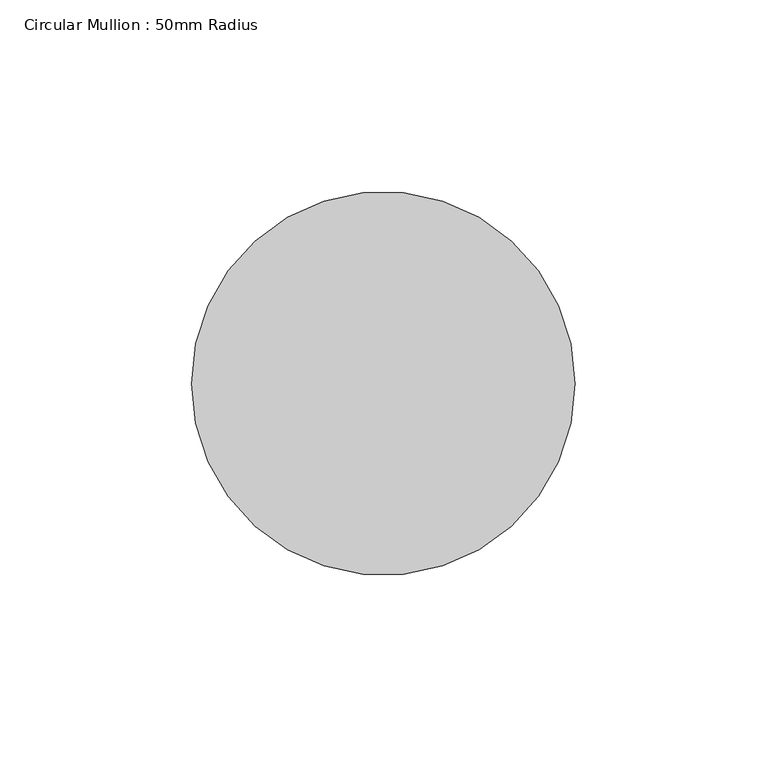
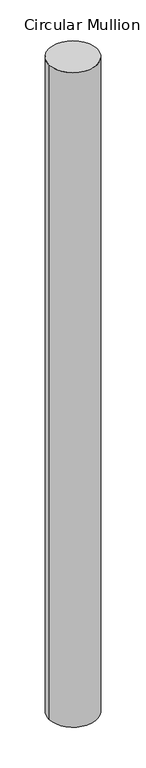
"""IFC4 building model written with IfcOpenShell, lengths in millimetres: member geometry, Circular Mullion : 50mm Radius."""

from ifc_helpers import new_model, si_unit, point, frame, origin, origin_2d, place, context, project, spatial, circle_curve, trimmed, segment, composite_curve, outline, extrude, source, transform, mapped, element, save


def circular_mullion_50mm_radius_7d129db9(model_context):
    return source(origin(), model_context, "Body", "SweptSolid", [
        extrude(outline(composite_curve([segment(trimmed(circle_curve(origin_2d(), 50.0), [point((50.0, 0.0))], [point((-50.0, 0.0))], False, "CARTESIAN"), True, "CONTINUOUS"), segment(trimmed(circle_curve(origin_2d(), 50.0), [point((-50.0, 0.0))], [point((50.0, 0.0))], False, "CARTESIAN"), True, "CONTINUOUS")], self_intersect=False)), frame((0.0, 0.0, -1433.6464214), z_axis=(0.0, 0.0, 1.0), x_axis=(1.0, 0.0, 0.0)), (0.0, 0.0, 1.0), 1433.6464214),
    ])


if __name__ == "__main__":
    model = new_model("IFC4")
    model_context = context("Model", 3, world=origin())
    ifc_project = project(units=[si_unit("LENGTHUNIT", "METRE", prefix="MILLI")], contexts=[model_context])
    site = spatial("IfcSite", under=ifc_project)
    building = spatial("IfcBuilding", under=site)
    placement = place(None, origin())
    circular_mullion_50mm_radius_shape = circular_mullion_50mm_radius_7d129db9(model_context)
    element("IfcMember", 1, ObjectType="Circular Mullion : 50mm Radius", at=placement, inside=building, context=model_context, shape_type="MappedRepresentation", body=[
        mapped(circular_mullion_50mm_radius_shape, transform((0.0, 0.0, 0.0), x_axis=(1.0, 0.0, 0.0), y_axis=(0.0, 1.0, 0.0), z_axis=(0.0, 0.0, 1.0))),
    ])
    save(model, "model.ifc")

# Revit data of these elements
# Type "Circular Mullion : 50mm Radius"
#   built-in parameter 1007350 = 0.164042 (stored number, unit not read)
# Element 1 (IfcMember, "Circular Mullion : 50mm Radius")
#   Materials on its faces: "Aluminium"
# Materials
#   "Aluminium": class "Metal", colour RGB 247 247 247, transparency 0, Description = "Aluminium 6061", Cost = 0
